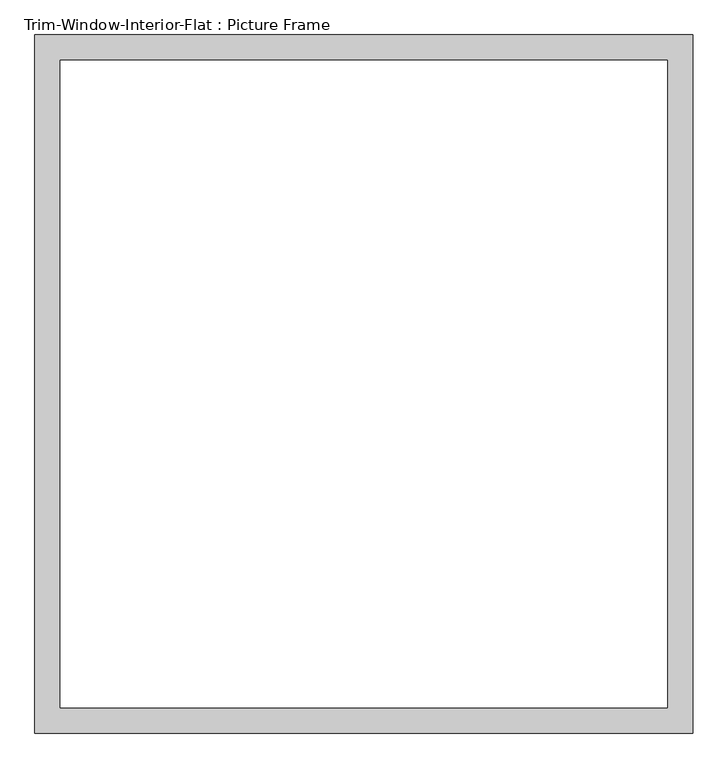
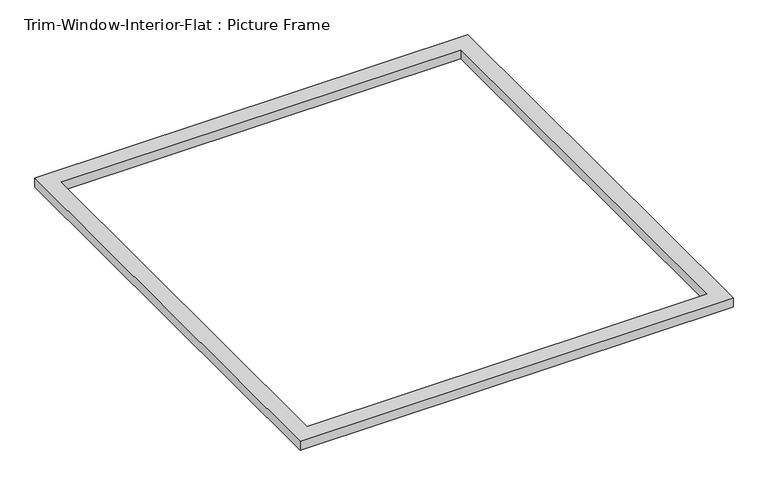
"""IFC4 building model written with IfcOpenShell, lengths in millimetres: proxy geometry, Trim-Window-Interior-Flat : Picture Frame."""

import ifcopenshell
import ifcopenshell.guid

model = None  # the IFC model being written
_history = None  # IfcOwnerHistory: only IFC2X3 demands one
_inside = {}  # id of a spatial element -> (the spatial element, [elements in it])
_under = {}  # id of a project, library or spatial element -> (it, [spatial elements below it])
_declared = {}  # id of a project -> (the project, [libraries it declares])
_typed = {}  # id of a type object -> (the type object, [elements of that type])
_made_of = {}  # id of a material, layer set ... -> (it, [elements and type objects made of it])


def new_model(schema):
    """Start an empty IFC model of exactly this schema.

    Asked for "IFC4X3", IfcOpenShell would pick the latest addendum, in which some entities
    have other attributes; the version numbers below select the first issue.
    IFC2X3 requires an IfcOwnerHistory on every rooted entity: one is made here for all.
    """
    global model, _history
    if schema == "IFC4X3":
        model = ifcopenshell.file(schema_version=(4, 3, 0, 0))
    else:
        model = ifcopenshell.file(schema=schema)
    _inside.clear()
    _under.clear()
    _declared.clear()
    _typed.clear()
    _made_of.clear()
    _history = None
    if model.schema == "IFC2X3":
        org = make("IfcOrganization", Name="unknown")
        user = make(
            "IfcPersonAndOrganization",
            ThePerson=make("IfcPerson", FamilyName="unknown"),
            TheOrganization=org,
        )
        app = make(
            "IfcApplication",
            ApplicationDeveloper=org,
            Version="unknown",
            ApplicationFullName="unknown",
            ApplicationIdentifier="unknown",
        )
        _history = make(
            "IfcOwnerHistory",
            OwningUser=user,
            OwningApplication=app,
            ChangeAction="ADDED",
            CreationDate=0,
        )
    return model


def make(cls, **values):
    """One entity of the class cls with the attributes given. An attribute that is None is left unset."""
    return model.create_entity(
        cls, **{name: value for name, value in values.items() if value is not None}
    )


def rooted(cls, **values):
    """An entity with a GlobalId (a new one), such as an element, a storey or a relation."""
    return make(cls, GlobalId=ifcopenshell.guid.new(), OwnerHistory=_history, **values)


def si_unit(unit_type, name, prefix=None):
    """IfcSIUnit, for example si_unit("LENGTHUNIT", "METRE", prefix="MILLI")."""
    return make("IfcSIUnit", UnitType=unit_type, Prefix=prefix, Name=name)


def assignment(units):
    """IfcUnitAssignment: the units of a project."""
    return None if units is None else make("IfcUnitAssignment", Units=units)


def point(xyz):
    """IfcCartesianPoint."""
    return None if xyz is None else make("IfcCartesianPoint", Coordinates=xyz)


def direction(xyz):
    """IfcDirection."""
    return None if xyz is None else make("IfcDirection", DirectionRatios=xyz)


def frame(location, z_axis=None, x_axis=None):
    """IfcAxis2Placement3D, a coordinate frame: its origin and axes. An axis left out is left unset."""
    return make(
        "IfcAxis2Placement3D",
        Location=point(location),
        Axis=direction(z_axis),
        RefDirection=direction(x_axis),
    )


def origin():
    """The frame at (0, 0, 0) with its axes left unset."""
    return frame((0.0, 0.0, 0.0))


def origin_with_axes():
    """The frame at (0, 0, 0) with the z axis (0, 0, 1) and the x axis (1, 0, 0) written out."""
    return frame((0.0, 0.0, 0.0), z_axis=(0.0, 0.0, 1.0), x_axis=(1.0, 0.0, 0.0))


def place(relative_to, where):
    """IfcLocalPlacement: puts the frame where relative to a parent placement (None: the world)."""
    return make(
        "IfcLocalPlacement", PlacementRelTo=relative_to, RelativePlacement=where
    )


def context(
    kind, dimensions, precision=None, world=None, true_north=None, identifier=None
):
    """IfcGeometricRepresentationContext, for example the 3D "Model" context."""
    return make(
        "IfcGeometricRepresentationContext",
        ContextIdentifier=identifier,
        ContextType=kind,
        CoordinateSpaceDimension=dimensions,
        Precision=precision,
        WorldCoordinateSystem=world,
        TrueNorth=true_north,
    )


def project(units=None, contexts=None):
    """IfcProject with its units and contexts."""
    return rooted(
        "IfcProject",
        Name="project",
        RepresentationContexts=contexts,
        UnitsInContext=assignment(units),
    )


def spatial(cls, under=None, at=None, **own):
    """A site, building, storey or space (cls), placed at a placement, below another one or the project."""
    s = rooted(cls, ObjectPlacement=at, **own)
    if under is not None:
        _under.setdefault(under.id(), (under, []))[1].append(s)
    return s


def polyline(points):
    """IfcPolyline through the points."""
    return make("IfcPolyline", Points=[point(p) for p in points])


def outline(outer, holes=None, kind="AREA"):
    """IfcArbitraryClosedProfileDef: a profile drawn as a closed curve; with holes, ...WithVoids."""
    if holes is None:
        return make("IfcArbitraryClosedProfileDef", ProfileType=kind, OuterCurve=outer)
    return make(
        "IfcArbitraryProfileDefWithVoids",
        ProfileType=kind,
        OuterCurve=outer,
        InnerCurves=holes,
    )


def extrude(swept, where, along, depth):
    """IfcExtrudedAreaSolid: the profile swept, set in the frame where, extruded along a direction by depth."""
    return make(
        "IfcExtrudedAreaSolid",
        SweptArea=swept,
        Position=where,
        ExtrudedDirection=direction(along),
        Depth=depth,
    )


def shape(context_of_items, identifier, shape_type, items):
    """IfcShapeRepresentation: the items that make up one representation, for example the "Body"."""
    return make(
        "IfcShapeRepresentation",
        ContextOfItems=context_of_items,
        RepresentationIdentifier=identifier,
        RepresentationType=shape_type,
        Items=items,
    )


def source(mapping_origin, context_of_items, identifier, shape_type, items):
    """IfcRepresentationMap: a shape defined once, which mapped items show again and again."""
    return make(
        "IfcRepresentationMap",
        MappingOrigin=mapping_origin,
        MappedRepresentation=shape(context_of_items, identifier, shape_type, items),
    )


def transform(
    local_origin,
    x_axis=None,
    y_axis=None,
    z_axis=None,
    scale=None,
    scale2=None,
    scale3=None,
    uniform=True,
):
    """IfcCartesianTransformationOperator3D, or its non-uniform kind. x_axis, y_axis, z_axis: its Axis1, 2, 3."""
    if uniform:
        return make(
            "IfcCartesianTransformationOperator3D",
            Axis1=direction(x_axis),
            Axis2=direction(y_axis),
            LocalOrigin=point(local_origin),
            Scale=scale,
            Axis3=direction(z_axis),
        )
    return make(
        "IfcCartesianTransformationOperator3DnonUniform",
        Axis1=direction(x_axis),
        Axis2=direction(y_axis),
        LocalOrigin=point(local_origin),
        Scale=scale,
        Axis3=direction(z_axis),
        Scale2=scale2,
        Scale3=scale3,
    )


def mapped(mapping_source, mapping_target):
    """IfcMappedItem: shows the shape of a source again, moved by a transform."""
    return make(
        "IfcMappedItem", MappingSource=mapping_source, MappingTarget=mapping_target
    )


def made_of(thing, what):
    """Note that an element or type object is made of a material, layer set ...; save() writes the relation."""
    if what is not None:
        _made_of.setdefault(what.id(), (what, []))[1].append(thing)
    return thing


def element(
    cls,
    number,
    at=None,
    inside=None,
    cuts=None,
    type_object=None,
    material=None,
    context=None,
    identifier="Body",
    shape_type=None,
    held_by="IfcProductDefinitionShape",
    body=None,
    shapes=None,
    **own,
):
    """One element of the class cls, such as IfcWall. Its Tag is "e" and its number.

    at: its placement. inside: the storey or other place that contains it. cuts: it is an
    opening in that element (IfcRelVoidsElement). A single representation is given by context,
    identifier, shape_type and body (its items); several are given by shapes. held_by: the class
    of the entity that holds the representations. save() writes the other relations.
    """
    e = rooted(cls, Tag="e%d" % number, ObjectPlacement=at, **own)
    if body is not None:
        shapes = [shape(context, identifier, shape_type, body)]
    if shapes is not None:
        e.Representation = make(held_by, Representations=shapes)
    if inside is not None:
        _inside.setdefault(inside.id(), (inside, []))[1].append(e)
    if cuts is not None:
        rooted(
            "IfcRelVoidsElement", RelatingBuildingElement=cuts, RelatedOpeningElement=e
        )
    if type_object is not None:
        _typed.setdefault(type_object.id(), (type_object, []))[1].append(e)
    return made_of(e, material)


def aggregate(whole, parts):
    """IfcRelAggregates: a whole, such as a stair, and the parts it consists of."""
    return rooted("IfcRelAggregates", RelatingObject=whole, RelatedObjects=parts)


def save(model, path):
    """Write the relations noted so far, then the file.

    IfcRelAggregates (storeys below a building ...), IfcRelContainedInSpatialStructure (elements
    in a storey), IfcRelDefinesByType, IfcRelAssociatesMaterial and IfcRelDeclares: one each for
    every whole, place, type object, material and project.
    """
    for whole, parts in _under.values():
        aggregate(whole, parts)
    for where, things in _inside.values():
        rooted(
            "IfcRelContainedInSpatialStructure",
            RelatedElements=things,
            RelatingStructure=where,
        )
    for kind, things in _typed.values():
        rooted("IfcRelDefinesByType", RelatedObjects=things, RelatingType=kind)
    for what, things in _made_of.values():
        rooted("IfcRelAssociatesMaterial", RelatedObjects=things, RelatingMaterial=what)
    for by, libraries in _declared.values():
        rooted("IfcRelDeclares", RelatingContext=by, RelatedDefinitions=libraries)
    model.write(path)


def trim_window_interior_flat_picture_frame_f9059606(model_context):
    return source(origin(), model_context, "Body", "SweptSolid", [
        extrude(outline(polyline([(736.6, 44.45), (736.6, -1517.65), (-736.6, -1517.65), (-736.6, 44.45), (736.6, 44.45)]), holes=[polyline([(679.45, -12.7), (-679.45, -12.7), (-679.45, -1460.5), (679.45, -1460.5), (679.45, -12.7)])]), origin_with_axes(), (0.0, 0.0, 1.0), 31.75),
    ])


if __name__ == "__main__":
    model = new_model("IFC4")
    model_context = context("Model", 3, world=origin())
    ifc_project = project(units=[si_unit("LENGTHUNIT", "METRE", prefix="MILLI")], contexts=[model_context])
    site = spatial("IfcSite", under=ifc_project)
    building = spatial("IfcBuilding", under=site)
    placement = place(None, origin())
    trim_window_interior_flat_picture_frame_shape = trim_window_interior_flat_picture_frame_f9059606(model_context)
    element("IfcBuildingElementProxy", 1, Name="Trim-Window-Interior-Flat : Picture Frame", ObjectType="Trim-Window-Interior-Flat : Picture Frame", at=placement, inside=building, context=model_context, shape_type="MappedRepresentation", body=[
        mapped(trim_window_interior_flat_picture_frame_shape, transform((0.0, 0.0, 0.0), x_axis=(1.0, 0.0, 0.0), y_axis=(0.0, 1.0, 0.0), z_axis=(0.0, 0.0, 1.0))),
    ])
    save(model, "model.ifc")

# Revit data of these elements
# Type "Trim-Window-Interior-Flat : Picture Frame"
#   Trim Thickness_Picture Frame = 0' - 1 1/4"
#   Trim Width = 0' - 2 1/4"
#   Trim Thickness_with Sill = 0' - 0 3/4"
#   Sill Thickness = 0' - 1 1/4"
#   Opening Width [instance default] = 2' - 0"
#   Opening Height [instance default] = 3' - 0"
#   Default Elevation = 4' - 0"
#   Sill = no
#   Picture Frame = yes
#   Trim Material [instance default] = none
# Element 1 (IfcBuildingElementProxy, "Trim-Window-Interior-Flat : Picture Frame")
#   Opening Width = 4' - 6 1/2"
#   Opening Height = 4' - 10"
#   Trim Material = Wood - Stained
#   Materials on its faces: "Wood - Stained"
# Materials
#   "Wood - Stained": class "Wood", colour RGB 224 178 126, transparency 0, Cost = 0
